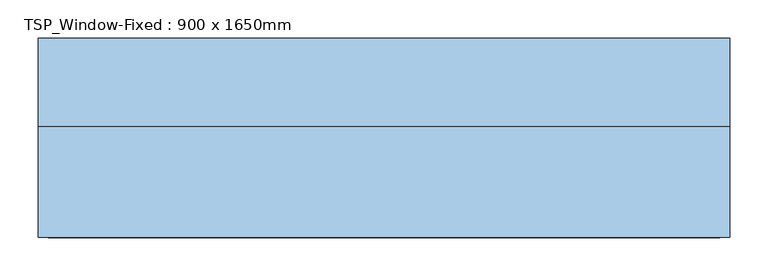
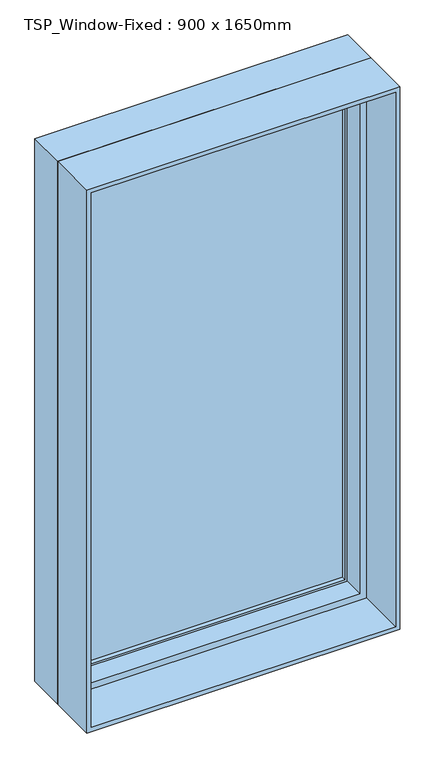
"""IFC4 building model written with IfcOpenShell, lengths in millimetres: window geometry, TSP_Window-Fixed : 900 x 1650mm."""

from ifc_helpers import new_model, si_unit, frame, origin, place, context, project, spatial, polyline, outline, extrude, faceted_brep, source, transform, mapped, element, save


def tsp_window_fixed_900_x_1650mm_17f2048f(model_context):
    return source(origin(), model_context, "Body", "SolidModel", [
        faceted_brep([(450.0, 24.75, 2550.0), (450.0, 139.05, 2550.0), (-450.0, 139.05, 2550.0), (-450.0, 24.75, 2550.0), (-450.0, 139.05, 900.0), (-450.0, 24.75, 900.0), (450.0, 139.05, 900.0), (450.0, 24.75, 900.0), (418.25, 24.75, 2518.25), (418.25, 24.75, 931.75), (-418.25, 24.75, 931.75), (-418.25, 24.75, 2518.25), (-437.3, 139.05, 2537.3), (-437.3, 139.05, 912.7), (437.3, 139.05, 912.7), (437.3, 139.05, 2537.3), (418.25, 88.25, 2518.25), (-418.25, 88.25, 2518.25), (437.3, 88.25, 2537.3), (-437.3, 88.25, 2537.3), (-418.25, 88.25, 931.75), (-437.3, 88.25, 912.7), (418.25, 88.25, 931.75), (437.3, 88.25, 912.7)], [[[0, 1, 2, 3]], [[3, 2, 4, 5]], [[5, 4, 6, 7]], [[3, 5, 7, 0], [8, 9, 10, 11]], [[7, 6, 1, 0]], [[1, 6, 4, 2], [12, 13, 14, 15]], [[16, 8, 11, 17]], [[15, 18, 19, 12]], [[17, 11, 10, 20]], [[12, 19, 21, 13]], [[20, 10, 9, 22]], [[13, 21, 23, 14]], [[22, 9, 8, 16]], [[18, 23, 21, 19], [17, 20, 22, 16]], [[14, 23, 18, 15]]]),
        extrude(outline(polyline([(2550.0, -450.0), (900.0, -450.0), (900.0, 450.0), (2550.0, 450.0), (2550.0, -450.0)]), holes=[polyline([(2537.3, 437.3), (912.7, 437.3), (912.7, -437.3), (2537.3, -437.3), (2537.3, 437.3)])]), frame((0.0, -120.0, 0.0), z_axis=(0.0, 1.0, 0.0), x_axis=(0.0, 0.0, 1.0)), (0.0, 0.0, 1.0), 144.75),
        extrude(outline(polyline([(912.7, 437.3), (2537.3, 437.3), (2537.3, -437.3), (912.7, -437.3), (912.7, 437.3)]), holes=[polyline([(938.1, -411.9), (2511.9, -411.9), (2511.9, 411.9), (938.1, 411.9), (938.1, -411.9)])]), frame((0.0, 88.25, 0.0), z_axis=(0.0, 1.0, 0.0), x_axis=(0.0, 0.0, 1.0)), (0.0, 0.0, 1.0), 44.45),
        extrude(outline(polyline([(411.9, 120.0), (411.9, 113.65), (-411.9, 113.65), (-411.9, 120.0), (411.9, 120.0)])), frame((0.0, 0.0, 938.1), z_axis=(0.0, 0.0, 1.0), x_axis=(1.0, 0.0, 0.0)), (0.0, 0.0, 1.0), 1573.8),
        extrude(outline(polyline([(-411.9, 100.95), (-411.9, 107.3), (411.9, 107.3), (411.9, 100.95), (-411.9, 100.95)])), frame((0.0, 0.0, 938.1), z_axis=(0.0, 0.0, 1.0), x_axis=(1.0, 0.0, 0.0)), (0.0, 0.0, 1.0), 1573.8),
    ])


if __name__ == "__main__":
    model = new_model("IFC4")
    model_context = context("Model", 3, world=origin())
    ifc_project = project(units=[si_unit("LENGTHUNIT", "METRE", prefix="MILLI")], contexts=[model_context])
    site = spatial("IfcSite", under=ifc_project)
    building = spatial("IfcBuilding", under=site)
    placement = place(None, origin())
    tsp_window_fixed_900_x_1650mm_shape = tsp_window_fixed_900_x_1650mm_17f2048f(model_context)
    element("IfcWindow", 1, ObjectType="TSP_Window-Fixed : 900 x 1650mm", at=placement, inside=building, context=model_context, shape_type="MappedRepresentation", body=[
        mapped(tsp_window_fixed_900_x_1650mm_shape, transform((0.0, 0.0, 0.0), x_axis=(1.0, 0.0, 0.0), y_axis=(0.0, 1.0, 0.0), z_axis=(0.0, 0.0, 1.0))),
    ])
    save(model, "model.ifc")

# Revit data of these elements
# Type "TSP_Window-Fixed : 900 x 1650mm"
#   Type Mark = "HS 2412 F153"
#   Fire Rating = "0.5h"
#   Assembly Code = "B2020100"
#   Analytic Construction = "Double glazing - domestic"
#   Window Inset [instance default] = 0 mm
#   Wall Thickness [instance default] = 150 mm
#   Visual Light Transmittance = 0.81
#   Thermal Resistance (R) = 0.319569 (m²·K)/W
#   Solar Heat Gain Coefficient = 0.76
#   Rough Width = 915 mm
#   Rough Height = 1665 mm
#   Interior Wall Closure [instance default] = 54.75 mm
#   Height = 1650 mm
#   Heat Transfer Coefficient (U) = 3.12929 W/(m²·K)
#   Frame Extension [instance default] = 6.35 mm
#   Exterior Wall Closure [instance default] = 31.75 mm
#   Extension Jamb [instance default] = 54.75 mm
#   Default Sill Height = 900 mm
#   Width = 900 mm
#   Muntin Visibility = yes
#   Interior Trim Visibility [instance default] = yes
#   Exterior Trim Visibility [instance default] = yes
#   Extension Jamb Visibility [instance default] = yes
#   Interior Trim Material = Wood - Stained
#   Interior Frame Material = Wood - Stained
#   Glass Panel Material = Glass
#   Exterior Trim Material = Clad - White
#   Exterior Frame Material = Clad - White
#   Wall Closure = (empty or 0)
# Element 1 (IfcWindow, "TSP_Window-Fixed : 900 x 1650mm")
#   Wall Thickness = 240 mm
#   Extension Jamb = 144.75 mm
#   Materials on its faces: "Wood - Stained", "Glass", "Clad - White"
# Materials
#   "Wood - Stained": class "Wood", colour RGB 224 178 126, transparency 0, Cost = 0
#   "Glass": class "Glass", colour RGB 0 128 192, transparency 0.9, Description = "Soda Lime Glass", Cost = 0
#   "Clad - White": class "Wood", colour RGB 242 242 238, transparency 0, Cost = 0
